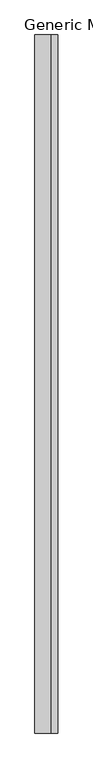
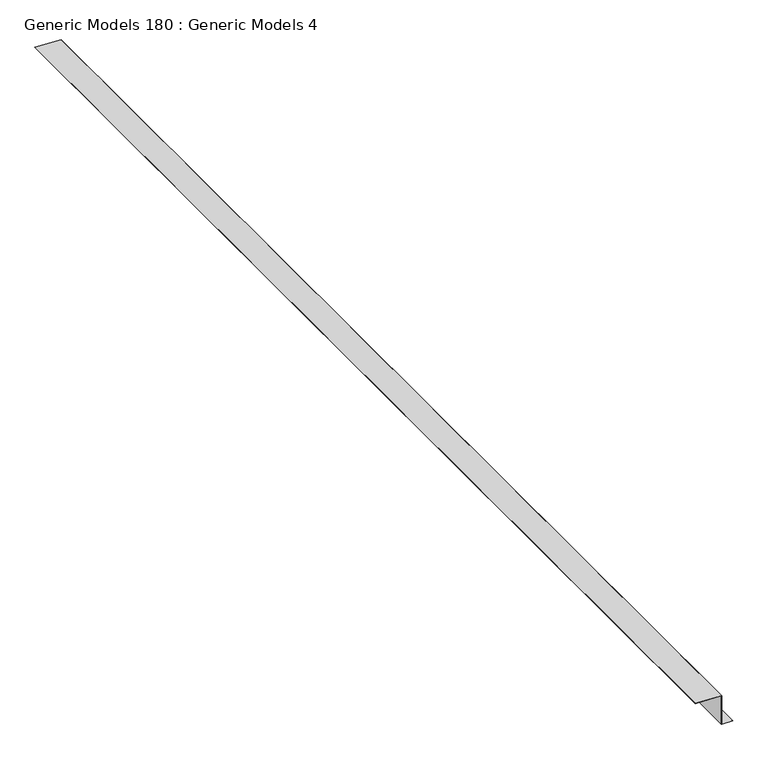
"""IFC4 building model written with IfcOpenShell, lengths in millimetres: proxy geometry, Generic Models 180 : Generic Models 4."""

from ifc_helpers import new_model, si_unit, frame, origin, place, context, project, spatial, polyline, outline, extrude, source, transform, mapped, element, save


def generic_models_180_generic_models_4_77bd5968(model_context):
    return source(origin(), model_context, "Body", "SweptSolid", [
        extrude(outline(polyline([(126922.824051, -8165.4798795), (126725.7567838, -8165.4798796), (126724.4431943, -8090.2243884), (126725.2368234, -8090.2105355), (126726.5367998, -8164.6861296), (126923.5855065, -8164.6861295), (126930.7706709, -8337.6195178), (126929.9776052, -8337.6524687), (126922.824051, -8165.4798795)])), frame((0.0, -464.1230338, 0.0), z_axis=(0.0, 1.0, 0.0), x_axis=(0.0, 0.0, 1.0)), (0.0, 0.0, 1.0), 7518.4),
    ])


if __name__ == "__main__":
    model = new_model("IFC4")
    model_context = context("Model", 3, world=origin())
    ifc_project = project(units=[si_unit("LENGTHUNIT", "METRE", prefix="MILLI")], contexts=[model_context])
    site = spatial("IfcSite", under=ifc_project)
    building = spatial("IfcBuilding", under=site)
    placement = place(None, origin())
    generic_models_180_generic_models_4_shape = generic_models_180_generic_models_4_77bd5968(model_context)
    element("IfcBuildingElementProxy", 1, Name="Generic Models 180 : Generic Models 4", ObjectType="Generic Models 180 : Generic Models 4", at=placement, inside=building, context=model_context, shape_type="MappedRepresentation", body=[
        mapped(generic_models_180_generic_models_4_shape, transform((0.0, 0.0, 0.0), x_axis=(1.0, 0.0, 0.0), y_axis=(0.0, 1.0, 0.0), z_axis=(0.0, 0.0, 1.0))),
    ])
    save(model, "model.ifc")

# Revit data of these elements
# Element 1 (IfcBuildingElementProxy, "Generic Models 180 : Generic Models 4")
#   Materials on its faces: "_HYDROSTOP LIQUID MEMBRANE -FOLLOW MANU. RECOMMENDED INSTALLATION DETAILS"
# Materials
#   "_HYDROSTOP LIQUID MEMBRANE -FOLLOW MANU. RECOMMENDED INSTALLATION DETAILS": class "Generic", colour RGB 100 140 119, transparency 0, Cost = 0
